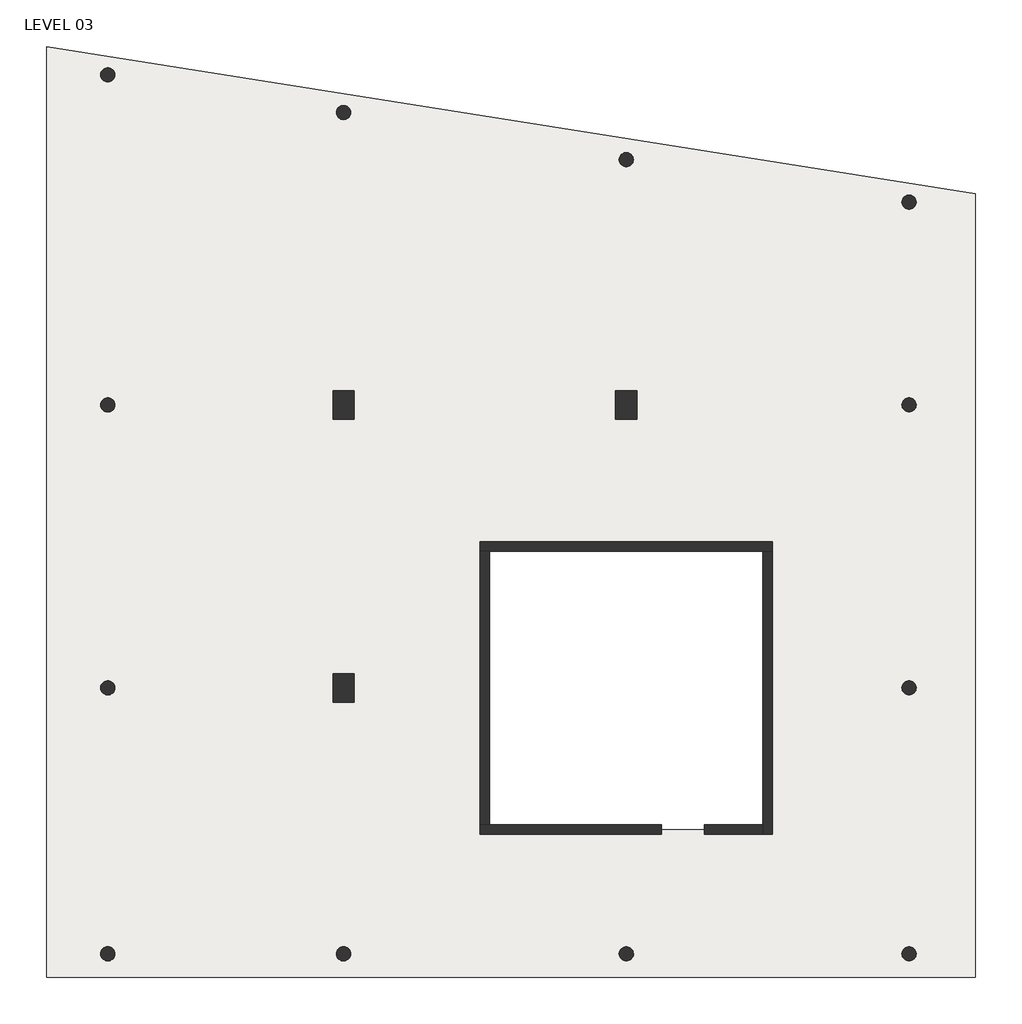
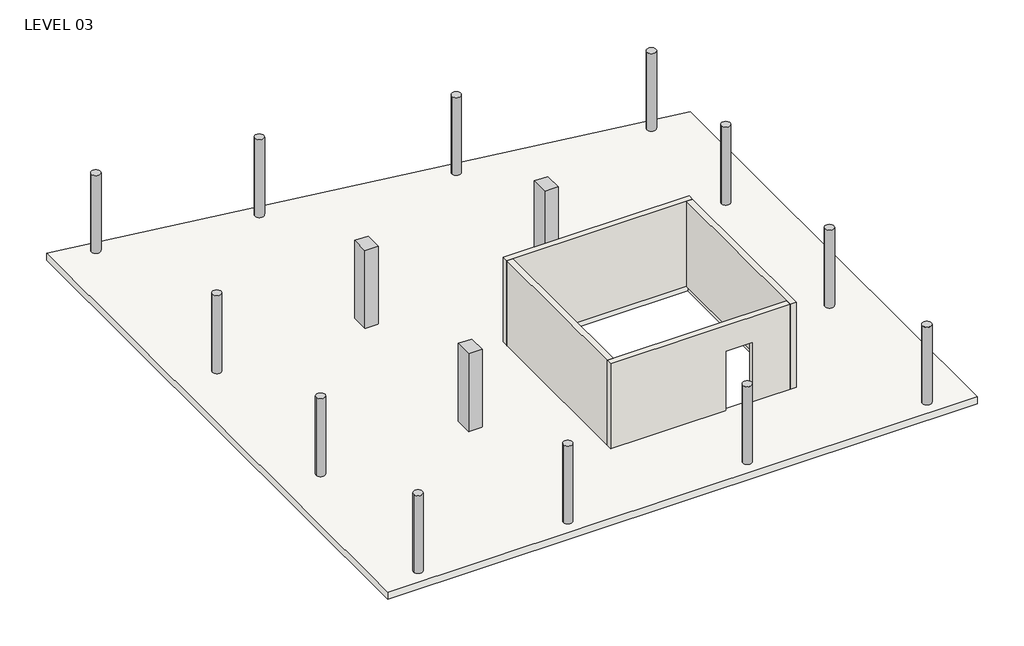
# One storey: 15 columns, 4 beams, 4 walls, 1 slab.
"""IFC4 building model written with IfcOpenShell, lengths in millimetres."""

from ifc_helpers import new_model, si_unit, point, frame, frame_2d, origin, place, context, project, spatial, polyline, circle_curve, trimmed, segment, composite_curve, outline, extrude, faceted_brep, element, save

model = new_model("IFC4")

# Units and contexts
model_context = context("Model", 3, world=origin())
ifc_project = project(units=[si_unit("LENGTHUNIT", "METRE", prefix="MILLI")], contexts=[model_context])

# Site, building, storey
site = spatial("IfcSite", under=ifc_project)
building = spatial("IfcBuilding", under=site)
storey = spatial("IfcBuildingStorey", under=building, Name="LEVEL 03", Elevation=9000.0)

# Beams
placement = place(None, origin())
element("IfcBeam", 1, ObjectType="BHm_StructuralFraming_Concrete-RectangularBeam : 300x500 DP RC BEAM", at=placement, inside=storey, context=model_context, shape_type="SweptSolid", body=[
    extrude(outline(composite_curve([segment(polyline([(-15925.1680269, 21640.7845261), (-15925.1680269, 14640.7845261)]), True, "CONTINUOUS"), segment(trimmed(circle_curve(frame_2d((-16075.1680269, 14640.7845261)), 150.0), [point((-15925.1680269, 14640.7845261))], [point((-16225.1680269, 14640.7845261))], True, "CARTESIAN"), True, "CONTINUOUS"), segment(polyline([(-16225.1680269, 14640.7845261), (-16225.1680269, 21640.7845261)]), True, "CONTINUOUS"), segment(trimmed(circle_curve(frame_2d((-16075.1680269, 21640.7845261)), 150.0), [point((-16225.1680269, 21640.7845261))], [point((-15925.1680269, 21640.7845261))], True, "CARTESIAN"), True, "CONTINUOUS")], self_intersect=False)), frame((0.0, 0.0, 8500.0), z_axis=(0.0, 0.0, 1.0), x_axis=(1.0, 0.0, 0.0)), (0.0, 0.0, 1.0), 250.0),
])
element("IfcBeam", 2, ObjectType="BHm_StructuralFraming_Concrete-RectangularBeam : 300x500 DP RC BEAM", at=placement, inside=storey, context=model_context, shape_type="SweptSolid", body=[
    extrude(outline(composite_curve([segment(polyline([(-10925.1680269, 20840.7845261), (-10925.1680269, 14940.7845261), (-11225.1680269, 14940.7845261), (-11225.1680269, 20840.7845261)]), True, "CONTINUOUS"), segment(trimmed(circle_curve(frame_2d((-11075.1680269, 20840.7845261)), 150.0), [point((-11225.1680269, 20840.7845261))], [point((-10925.1680269, 20840.7845261))], True, "CARTESIAN"), True, "CONTINUOUS")], self_intersect=False)), frame((0.0, 0.0, 8500.0), z_axis=(0.0, 0.0, 1.0), x_axis=(1.0, 0.0, 0.0)), (0.0, 0.0, 1.0), 250.0),
])
element("IfcBeam", 3, ObjectType="BHm_StructuralFraming_Concrete-RectangularBeam : 300x500 DP RC BEAM", at=placement, inside=storey, context=model_context, shape_type="SweptSolid", body=[
    extrude(outline(composite_curve([segment(polyline([(-4925.1680269, 19840.7845261), (-4925.1680269, 14940.7845261), (-5225.1680269, 14940.7845261), (-5225.1680269, 19840.7845261)]), True, "CONTINUOUS"), segment(trimmed(circle_curve(frame_2d((-5075.1680269, 19840.7845261)), 150.0), [point((-5225.1680269, 19840.7845261))], [point((-4925.1680269, 19840.7845261))], True, "CARTESIAN"), True, "CONTINUOUS")], self_intersect=False)), frame((0.0, 0.0, 8500.0), z_axis=(0.0, 0.0, 1.0), x_axis=(1.0, 0.0, 0.0)), (0.0, 0.0, 1.0), 250.0),
])
element("IfcBeam", 4, ObjectType="BHm_StructuralFraming_Concrete-RectangularBeam : 300x500 DP RC BEAM", at=placement, inside=storey, context=model_context, shape_type="SweptSolid", body=[
    extrude(outline(composite_curve([segment(polyline([(1074.8319731, 18940.7845261), (1074.8319731, 14640.7845261)]), True, "CONTINUOUS"), segment(trimmed(circle_curve(frame_2d((924.8319731, 14640.7845261)), 150.0), [point((1074.8319731, 14640.7845261))], [point((774.8319731, 14640.7845261))], True, "CARTESIAN"), True, "CONTINUOUS"), segment(polyline([(774.8319731, 14640.7845261), (774.8319731, 18940.7845261)]), True, "CONTINUOUS"), segment(trimmed(circle_curve(frame_2d((924.8319731, 18940.7845261)), 150.0), [point((774.8319731, 18940.7845261))], [point((1074.8319731, 18940.7845261))], True, "CARTESIAN"), True, "CONTINUOUS")], self_intersect=False)), frame((0.0, 0.0, 8500.0), z_axis=(0.0, 0.0, 1.0), x_axis=(1.0, 0.0, 0.0)), (0.0, 0.0, 1.0), 250.0),
])

# Columns
element("IfcColumn", 5, ObjectType="BHm_StructuralColumns_ConcreteRound : 300 Ø RC COL", at=placement, inside=storey, context=model_context, shape_type="SweptSolid", body=[
    extrude(outline(composite_curve([segment(trimmed(circle_curve(frame_2d((-5075.1680269, 3000.0)), 150.0), [point((-5225.1680269, 3000.0))], [point((-4925.1680269, 3000.0))], False, "CARTESIAN"), True, "CONTINUOUS"), segment(trimmed(circle_curve(frame_2d((-5075.1680269, 3000.0)), 150.0), [point((-4925.1680269, 3000.0))], [point((-5225.1680269, 3000.0))], False, "CARTESIAN"), True, "CONTINUOUS")], self_intersect=False)), frame((0.0, 0.0, 9000.0), z_axis=(0.0, 0.0, 1.0), x_axis=(1.0, 0.0, 0.0)), (0.0, 0.0, 1.0), 2750.0),
])
element("IfcColumn", 6, ObjectType="BHm_StructuralColumns_ConcreteRound : 300 Ø RC COL", at=placement, inside=storey, context=model_context, shape_type="SweptSolid", body=[
    extrude(outline(composite_curve([segment(trimmed(circle_curve(frame_2d((924.8319731, 14640.7845261)), 150.0), [point((774.8319731, 14640.7845261))], [point((1074.8319731, 14640.7845261))], False, "CARTESIAN"), True, "CONTINUOUS"), segment(trimmed(circle_curve(frame_2d((924.8319731, 14640.7845261)), 150.0), [point((1074.8319731, 14640.7845261))], [point((774.8319731, 14640.7845261))], False, "CARTESIAN"), True, "CONTINUOUS")], self_intersect=False)), frame((0.0, 0.0, 9000.0), z_axis=(0.0, 0.0, 1.0), x_axis=(1.0, 0.0, 0.0)), (0.0, 0.0, 1.0), 2750.0),
])
element("IfcColumn", 7, ObjectType="BHm_StructuralColumns_ConcreteRound : 300 Ø RC COL", at=placement, inside=storey, context=model_context, shape_type="SweptSolid", body=[
    extrude(outline(composite_curve([segment(trimmed(circle_curve(frame_2d((924.8319731, 8640.7845261)), 150.0), [point((774.8319731, 8640.7845261))], [point((1074.8319731, 8640.7845261))], False, "CARTESIAN"), True, "CONTINUOUS"), segment(trimmed(circle_curve(frame_2d((924.8319731, 8640.7845261)), 150.0), [point((1074.8319731, 8640.7845261))], [point((774.8319731, 8640.7845261))], False, "CARTESIAN"), True, "CONTINUOUS")], self_intersect=False)), frame((0.0, 0.0, 9000.0), z_axis=(0.0, 0.0, 1.0), x_axis=(1.0, 0.0, 0.0)), (0.0, 0.0, 1.0), 2750.0),
])
element("IfcColumn", 8, ObjectType="BHm_StructuralColumns_ConcreteRound : 300 Ø RC COL", at=placement, inside=storey, context=model_context, shape_type="SweptSolid", body=[
    extrude(outline(composite_curve([segment(trimmed(circle_curve(frame_2d((924.8319731, 3000.0)), 150.0), [point((774.8319731, 3000.0))], [point((1074.8319731, 3000.0))], False, "CARTESIAN"), True, "CONTINUOUS"), segment(trimmed(circle_curve(frame_2d((924.8319731, 3000.0)), 150.0), [point((1074.8319731, 3000.0))], [point((774.8319731, 3000.0))], False, "CARTESIAN"), True, "CONTINUOUS")], self_intersect=False)), frame((0.0, 0.0, 9000.0), z_axis=(0.0, 0.0, 1.0), x_axis=(1.0, 0.0, 0.0)), (0.0, 0.0, 1.0), 2750.0),
])
element("IfcColumn", 9, ObjectType="BHm_StructuralColumns_ConcreteRound : 300 Ø RC COL", at=placement, inside=storey, context=model_context, shape_type="SweptSolid", body=[
    extrude(outline(composite_curve([segment(trimmed(circle_curve(frame_2d((-11075.1680269, 3000.0)), 150.0), [point((-11225.1680269, 3000.0))], [point((-10925.1680269, 3000.0))], False, "CARTESIAN"), True, "CONTINUOUS"), segment(trimmed(circle_curve(frame_2d((-11075.1680269, 3000.0)), 150.0), [point((-10925.1680269, 3000.0))], [point((-11225.1680269, 3000.0))], False, "CARTESIAN"), True, "CONTINUOUS")], self_intersect=False)), frame((0.0, 0.0, 9000.0), z_axis=(0.0, 0.0, 1.0), x_axis=(1.0, 0.0, 0.0)), (0.0, 0.0, 1.0), 2750.0),
])
element("IfcColumn", 10, ObjectType="BHm_StructuralColumns_ConcreteRound : 300 Ø RC COL", at=placement, inside=storey, context=model_context, shape_type="SweptSolid", body=[
    extrude(outline(composite_curve([segment(trimmed(circle_curve(frame_2d((-16075.1680269, 14640.7845261)), 150.0), [point((-16225.1680269, 14640.7845261))], [point((-15925.1680269, 14640.7845261))], False, "CARTESIAN"), True, "CONTINUOUS"), segment(trimmed(circle_curve(frame_2d((-16075.1680269, 14640.7845261)), 150.0), [point((-15925.1680269, 14640.7845261))], [point((-16225.1680269, 14640.7845261))], False, "CARTESIAN"), True, "CONTINUOUS")], self_intersect=False)), frame((0.0, 0.0, 9000.0), z_axis=(0.0, 0.0, 1.0), x_axis=(1.0, 0.0, 0.0)), (0.0, 0.0, 1.0), 2750.0),
])
element("IfcColumn", 11, ObjectType="BHm_StructuralColumns_ConcreteRound : 300 Ø RC COL", at=placement, inside=storey, context=model_context, shape_type="SweptSolid", body=[
    extrude(outline(composite_curve([segment(trimmed(circle_curve(frame_2d((-16075.1680269, 8640.7845261)), 150.0), [point((-16225.1680269, 8640.7845261))], [point((-15925.1680269, 8640.7845261))], False, "CARTESIAN"), True, "CONTINUOUS"), segment(trimmed(circle_curve(frame_2d((-16075.1680269, 8640.7845261)), 150.0), [point((-15925.1680269, 8640.7845261))], [point((-16225.1680269, 8640.7845261))], False, "CARTESIAN"), True, "CONTINUOUS")], self_intersect=False)), frame((0.0, 0.0, 9000.0), z_axis=(0.0, 0.0, 1.0), x_axis=(1.0, 0.0, 0.0)), (0.0, 0.0, 1.0), 2750.0),
])
element("IfcColumn", 12, ObjectType="BHm_StructuralColumns_ConcreteRound : 300 Ø RC COL", at=placement, inside=storey, context=model_context, shape_type="SweptSolid", body=[
    extrude(outline(composite_curve([segment(trimmed(circle_curve(frame_2d((-16075.1680269, 3000.0)), 150.0), [point((-16225.1680269, 3000.0))], [point((-15925.1680269, 3000.0))], False, "CARTESIAN"), True, "CONTINUOUS"), segment(trimmed(circle_curve(frame_2d((-16075.1680269, 3000.0)), 150.0), [point((-15925.1680269, 3000.0))], [point((-16225.1680269, 3000.0))], False, "CARTESIAN"), True, "CONTINUOUS")], self_intersect=False)), frame((0.0, 0.0, 9000.0), z_axis=(0.0, 0.0, 1.0), x_axis=(1.0, 0.0, 0.0)), (0.0, 0.0, 1.0), 2750.0),
])
element("IfcColumn", 13, ObjectType="BHm_StructuralColumns_ConcreteRound : 300 Ø RC COL", at=placement, inside=storey, context=model_context, shape_type="SweptSolid", body=[
    extrude(outline(composite_curve([segment(trimmed(circle_curve(frame_2d((-11075.1680269, 20840.7845261)), 150.0), [point((-11225.1680269, 20840.7845261))], [point((-10925.1680269, 20840.7845261))], False, "CARTESIAN"), True, "CONTINUOUS"), segment(trimmed(circle_curve(frame_2d((-11075.1680269, 20840.7845261)), 150.0), [point((-10925.1680269, 20840.7845261))], [point((-11225.1680269, 20840.7845261))], False, "CARTESIAN"), True, "CONTINUOUS")], self_intersect=False)), frame((0.0, 0.0, 9000.0), z_axis=(0.0, 0.0, 1.0), x_axis=(1.0, 0.0, 0.0)), (0.0, 0.0, 1.0), 2750.0),
])
element("IfcColumn", 14, ObjectType="BHm_StructuralColumns_ConcreteRound : 300 Ø RC COL", at=placement, inside=storey, context=model_context, shape_type="SweptSolid", body=[
    extrude(outline(composite_curve([segment(trimmed(circle_curve(frame_2d((-5075.1680269, 19840.7845261)), 150.0), [point((-5225.1680269, 19840.7845261))], [point((-4925.1680269, 19840.7845261))], False, "CARTESIAN"), True, "CONTINUOUS"), segment(trimmed(circle_curve(frame_2d((-5075.1680269, 19840.7845261)), 150.0), [point((-4925.1680269, 19840.7845261))], [point((-5225.1680269, 19840.7845261))], False, "CARTESIAN"), True, "CONTINUOUS")], self_intersect=False)), frame((0.0, 0.0, 9000.0), z_axis=(0.0, 0.0, 1.0), x_axis=(1.0, 0.0, 0.0)), (0.0, 0.0, 1.0), 2750.0),
])
element("IfcColumn", 15, ObjectType="BHm_StructuralColumns_ConcreteRound : 300 Ø RC COL", at=placement, inside=storey, context=model_context, shape_type="SweptSolid", body=[
    extrude(outline(composite_curve([segment(trimmed(circle_curve(frame_2d((924.8319731, 18940.7845261)), 150.0), [point((774.8319731, 18940.7845261))], [point((1074.8319731, 18940.7845261))], False, "CARTESIAN"), True, "CONTINUOUS"), segment(trimmed(circle_curve(frame_2d((924.8319731, 18940.7845261)), 150.0), [point((1074.8319731, 18940.7845261))], [point((774.8319731, 18940.7845261))], False, "CARTESIAN"), True, "CONTINUOUS")], self_intersect=False)), frame((0.0, 0.0, 9000.0), z_axis=(0.0, 0.0, 1.0), x_axis=(1.0, 0.0, 0.0)), (0.0, 0.0, 1.0), 2750.0),
])
element("IfcColumn", 16, ObjectType="BHm_StructuralColumns_ConcreteRound : 300 Ø RC COL", at=placement, inside=storey, context=model_context, shape_type="SweptSolid", body=[
    extrude(outline(composite_curve([segment(trimmed(circle_curve(frame_2d((-16075.1680269, 21640.7845261)), 150.0), [point((-16225.1680269, 21640.7845261))], [point((-15925.1680269, 21640.7845261))], False, "CARTESIAN"), True, "CONTINUOUS"), segment(trimmed(circle_curve(frame_2d((-16075.1680269, 21640.7845261)), 150.0), [point((-15925.1680269, 21640.7845261))], [point((-16225.1680269, 21640.7845261))], False, "CARTESIAN"), True, "CONTINUOUS")], self_intersect=False)), frame((0.0, 0.0, 9000.0), z_axis=(0.0, 0.0, 1.0), x_axis=(1.0, 0.0, 0.0)), (0.0, 0.0, 1.0), 2750.0),
])
element("IfcColumn", 17, ObjectType="BHm_StructuralColumns_ConcreteRectangular : 450x600 RC COL", at=placement, inside=storey, context=model_context, shape_type="SweptSolid", body=[
    extrude(outline(polyline([(-10850.1680269, 14940.7845261), (-10850.1680269, 14340.7845261), (-11300.1680269, 14340.7845261), (-11300.1680269, 14940.7845261), (-10850.1680269, 14940.7845261)])), frame((0.0, 0.0, 9000.0), z_axis=(0.0, 0.0, 1.0), x_axis=(1.0, 0.0, 0.0)), (0.0, 0.0, 1.0), 2750.0),
])
element("IfcColumn", 18, ObjectType="BHm_StructuralColumns_ConcreteRectangular : 450x600 RC COL", at=placement, inside=storey, context=model_context, shape_type="SweptSolid", body=[
    extrude(outline(polyline([(-10850.1680269, 8940.7845261), (-10850.1680269, 8340.7845261), (-11300.1680269, 8340.7845261), (-11300.1680269, 8940.7845261), (-10850.1680269, 8940.7845261)])), frame((0.0, 0.0, 9000.0), z_axis=(0.0, 0.0, 1.0), x_axis=(1.0, 0.0, 0.0)), (0.0, 0.0, 1.0), 2750.0),
])
element("IfcColumn", 19, ObjectType="BHm_StructuralColumns_ConcreteRectangular : 450x600 RC COL", at=placement, inside=storey, context=model_context, shape_type="SweptSolid", body=[
    extrude(outline(polyline([(-4850.1680269, 14940.7845261), (-4850.1680269, 14340.7845261), (-5300.1680269, 14340.7845261), (-5300.1680269, 14940.7845261), (-4850.1680269, 14940.7845261)])), frame((0.0, 0.0, 9000.0), z_axis=(0.0, 0.0, 1.0), x_axis=(1.0, 0.0, 0.0)), (0.0, 0.0, 1.0), 2750.0),
])

# Slab
element("IfcSlab", 20, ObjectType="250 THK RC SLAB", at=placement, inside=storey, context=model_context, shape_type="SweptSolid", body=[
    extrude(outline(polyline([(2324.8319731, 19120.6110517), (2324.8319731, 2500.0), (-17375.1680269, 2500.0), (-17375.1680269, 22240.7845261), (2324.8319731, 19120.6110517)]), holes=[polyline([(-2075.1680269, 11640.7845261), (-8075.1680269, 11640.7845261), (-8075.1680269, 5640.7845261), (-2075.1680269, 5640.7845261), (-2075.1680269, 11640.7845261)])]), frame((0.0, 0.0, 8750.0), z_axis=(0.0, 0.0, 1.0), x_axis=(1.0, 0.0, 0.0)), (0.0, 0.0, 1.0), 250.0),
])

# Walls
element("IfcWall", 21, ObjectType="200 THK R.C. WALL", at=placement, inside=storey, context=model_context, shape_type="Brep", body=[
    faceted_brep([(-8175.1680269, 11540.7845261, 9000.0), (-7975.1680269, 11540.7845261, 9000.0), (-2175.1680269, 11540.7845261, 9000.0), (-1975.1680269, 11540.7845261, 9000.0), (-1975.1680269, 11540.7845261, 12000.0), (-2175.1680269, 11540.7845261, 12000.0), (-7975.1680269, 11540.7845261, 12000.0), (-8175.1680269, 11540.7845261, 12000.0), (-8175.1680269, 11740.7845261, 9000.0), (-8175.1680269, 11740.7845261, 12000.0), (-1975.1680269, 11740.7845261, 12000.0), (-1975.1680269, 11740.7845261, 9000.0)], [[[0, 1, 2, 3, 4, 5, 6, 7]], [[8, 9, 10, 11]], [[3, 2, 1, 0, 8, 11]], [[7, 6, 5, 4, 10, 9]], [[4, 3, 11, 10]], [[0, 7, 9, 8]]]),
])
element("IfcWall", 22, ObjectType="200 THK R.C. WALL", at=placement, inside=storey, context=model_context, shape_type="Brep", body=[
    faceted_brep([(-2175.1680269, 11540.7845261, 9000.0), (-2175.1680269, 5740.7845261, 9000.0), (-2175.1680269, 5540.7845261, 9000.0), (-2175.1680269, 5540.7845261, 12000.0), (-2175.1680269, 5740.7845261, 12000.0), (-2175.1680269, 11540.7845261, 12000.0), (-1975.1680269, 11540.7845261, 9000.0), (-1975.1680269, 11540.7845261, 12000.0), (-1975.1680269, 5540.7845261, 12000.0), (-1975.1680269, 5540.7845261, 9000.0)], [[[0, 1, 2, 3, 4, 5]], [[6, 7, 8, 9]], [[2, 1, 0, 6, 9]], [[5, 4, 3, 8, 7]], [[0, 5, 7, 6]], [[3, 2, 9, 8]]]),
])
element("IfcWall", 23, ObjectType="200 THK R.C. WALL", at=placement, inside=storey, context=model_context, shape_type="Brep", body=[
    faceted_brep([(-2175.1680269, 5740.7845261, 9000.0), (-3417.6680269, 5740.7845261, 9000.0), (-3417.6680269, 5740.7845261, 11100.0), (-4332.6680269, 5740.7845261, 11100.0), (-4332.6680269, 5740.7845261, 9000.0), (-7975.1680269, 5740.7845261, 9000.0), (-8175.1680269, 5740.7845261, 9000.0), (-8175.1680269, 5740.7845261, 12000.0), (-7975.1680269, 5740.7845261, 12000.0), (-2175.1680269, 5740.7845261, 12000.0), (-3417.6680269, 5540.7845261, 11100.0), (-3417.6680269, 5540.7845261, 9000.0), (-2175.1680269, 5540.7845261, 9000.0), (-2175.1680269, 5540.7845261, 12000.0), (-8175.1680269, 5540.7845261, 12000.0), (-8175.1680269, 5540.7845261, 9000.0), (-4332.6680269, 5540.7845261, 9000.0), (-4332.6680269, 5540.7845261, 11100.0)], [[[0, 1, 2, 3, 4, 5, 6, 7, 8, 9]], [[10, 11, 12, 13, 14, 15, 16, 17]], [[16, 15, 6, 5, 4]], [[12, 11, 1, 0]], [[9, 8, 7, 14, 13]], [[0, 9, 13, 12]], [[7, 6, 15, 14]], [[4, 3, 17, 16]], [[2, 1, 11, 10]], [[3, 2, 10, 17]]]),
])
element("IfcWall", 24, ObjectType="200 THK R.C. WALL", at=placement, inside=storey, context=model_context, shape_type="SweptSolid", body=[
    extrude(outline(polyline([(-7975.1680269, 11540.7845261), (-7975.1680269, 5740.7845261), (-8175.1680269, 5740.7845261), (-8175.1680269, 11540.7845261), (-7975.1680269, 11540.7845261)])), frame((0.0, 0.0, 9000.0), z_axis=(0.0, 0.0, 1.0), x_axis=(1.0, 0.0, 0.0)), (0.0, 0.0, 1.0), 3000.0),
])

save(model, "model.ifc")

# Revit data of these elements
# Type "BHm_StructuralFraming_Concrete-RectangularBeam : 300x500 DP RC BEAM"
#   Keynote = "E"
#   BHE_Width = 300.000 mm
#   BHE_Length [instance default] = 1524.000 mm
#   BHE_Height = 500.000 mm
#   Length [instance default] = 1524.000 mm
#   b = 300.000 mm
#   h = 500.000 mm
#   Structural Material [instance default] = none
#   Assembly Code = ""
# Type "BHm_StructuralColumns_ConcreteRound : 300 Ø RC COL"
#   Keynote = "E"
#   b = 300.000 mm
#   BHE_Length [instance default] = 2500.000 mm
#   BHE_Diameter = 300.000 mm
#   Structural Material [instance default] = none
# Type "BHm_StructuralColumns_ConcreteRectangular : 450x600 RC COL"
#   Keynote = "E"
#   b = 450.000 mm
#   h = 600.000 mm
#   BHE_Width = 450.000 mm
#   BHE_Length [instance default] = 2500.000 mm
#   BHE_Height = 600.000 mm
#   Structural Material [instance default] = none
# Type "250 THK RC SLAB"
#   Function = 0
#   Layers, outside or top first: 250.000 mm "BHE_Concrete - Cast In-Place" (function 1)
# Type "200 THK R.C. WALL"
#   Layers, outside or top first: 200.000 mm "BHE_Concrete - Cast In-Place" (function 1)
# Element 1 (IfcBeam, "BHm_StructuralFraming_Concrete-RectangularBeam : 300x500 DP RC BEAM")
#   Comments = ""
#   BHE_Length = 7000.000 mm
#   Structural Material = none
#   Phase Created = New Construction
#   Materials on its faces: "BHE_Concrete - Cast In-Place"
# Element 2 (IfcBeam, "BHm_StructuralFraming_Concrete-RectangularBeam : 300x500 DP RC BEAM")
#   Comments = ""
#   BHE_Length = 6200.000 mm
#   Structural Material = none
#   Phase Created = New Construction
#   Materials on its faces: "BHE_Concrete - Cast In-Place"
# Element 3 (IfcBeam, "BHm_StructuralFraming_Concrete-RectangularBeam : 300x500 DP RC BEAM")
#   Comments = ""
#   BHE_Length = 5200.000 mm
#   Structural Material = none
#   Phase Created = New Construction
#   Materials on its faces: "BHE_Concrete - Cast In-Place"
# Element 4 (IfcBeam, "BHm_StructuralFraming_Concrete-RectangularBeam : 300x500 DP RC BEAM")
#   Comments = ""
#   BHE_Length = 4300.000 mm
#   Structural Material = none
#   Phase Created = New Construction
#   Materials on its faces: "BHE_Concrete - Cast In-Place"
# Elements 5, 6, 7, 8, 9, 10, 11, 12, 13, 14, 15, 16 (IfcColumn, "BHm_StructuralColumns_ConcreteRound : 300 Ø RC COL")
#   Comments = ""
#   Structural Material = none
#   Phase Created = New Construction
#   Materials on its faces: "BHE_Concrete - Cast In-Place"
# Elements 17, 18, 19 (IfcColumn, "BHm_StructuralColumns_ConcreteRectangular : 450x600 RC COL")
#   Comments = ""
#   Structural Material = none
#   Phase Created = New Construction
#   Materials on its faces: "BHE_Concrete - Cast In-Place"
# Element 20 (IfcSlab, "250 THK RC SLAB")
#   Comments = ""
#   built-in parameter 1001955 = -0.15708 (stored number, unit not read)
#   Height Offset From Level = 0.000 mm
#   built-in parameter 1001954 = 1
#   Phase Created = New Construction
#   Materials on its faces: "BHE_Concrete - Cast In-Place"
# Elements 21, 22, 23, 24 (IfcWall, "200 THK R.C. WALL")
#   Comments = ""
#   Top Offset = 0.000 mm
#   Base Offset = 0.000 mm
#   wall height = 3000.000 mm
#   Phase Created = New Construction
#   Base Constraint = LEVEL 03
#   Top Constraint = LEVEL 04
#   Materials on its faces: "BHE_Concrete - Cast In-Place"
# Materials
#   "BHE_Concrete - Cast In-Place": class "Concrete", colour RGB 192 192 192, transparency 0, Cost = 0
